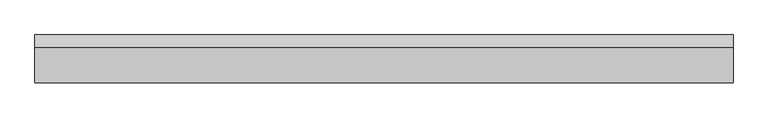
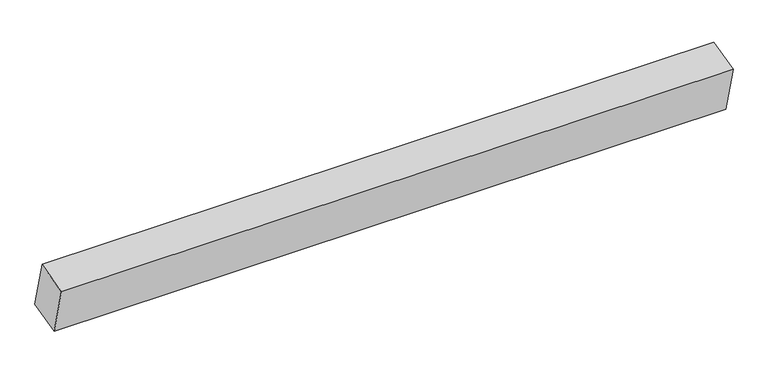
"""IFC4 building model written with IfcOpenShell, lengths in millimetres: proxy geometry, Insulation010 1090 : Insulation010 1090."""

from ifc_helpers import new_model, si_unit, frame, origin, place, context, project, spatial, polyline, outline, extrude, source, transform, mapped, element, save


def generic_models_1bb2289c(model_context):
    return source(origin(), model_context, "Body", "SweptSolid", [
        extrude(outline(polyline([(9725.8093592, 43266.8523503), (9625.78052, 43241.8381723), (9588.8164512, 43389.6944477), (9688.8469299, 43414.7020673), (9725.8093592, 43266.8523503)])), frame((3694.2883192, 0.0, 0.0), z_axis=(1.0, 0.0, 0.0), x_axis=(0.0, 1.0, 0.0)), (0.0, 0.0, 1.0), 2000.0),
    ])


if __name__ == "__main__":
    model = new_model("IFC4")
    model_context = context("Model", 3, world=origin())
    ifc_project = project(units=[si_unit("LENGTHUNIT", "METRE", prefix="MILLI")], contexts=[model_context])
    site = spatial("IfcSite", under=ifc_project)
    building = spatial("IfcBuilding", under=site)
    placement = place(None, origin())
    generic_models_shape = generic_models_1bb2289c(model_context)
    element("IfcBuildingElementProxy", 1, Name="Insulation010 1090 : Insulation010 1090", ObjectType="Insulation010 1090 : Insulation010 1090", at=placement, inside=building, context=model_context, shape_type="MappedRepresentation", body=[
        mapped(generic_models_shape, transform((0.0, 0.0, 0.0), x_axis=(1.0, 0.0, 0.0), y_axis=(0.0, 1.0, 0.0), z_axis=(0.0, 0.0, 1.0))),
    ])
    save(model, "model.ifc")

# Revit data of these elements
# Type "Insulation010 1090 : Insulation010 1090"
#   NameOverride = "Insulation010"
# Element 1 (IfcBuildingElementProxy, "Insulation010 1090 : Insulation010 1090")
#   Materials on its faces: "BATT INSULATION (U-FACTOR = 0.065 MIN.) OVER CLASS II VAPOR RETARDER (TOWARDS INTERIOR)"
# Materials
#   "BATT INSULATION (U-FACTOR = 0.065 MIN.) OVER CLASS II VAPOR RETARDER (TOWARDS INTERIOR)": class "Unassigned", colour RGB 246 242 160, transparency 0, Cost = 0
